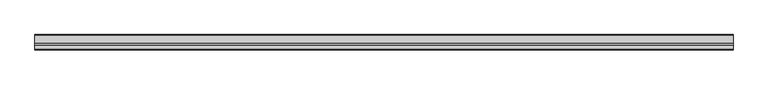
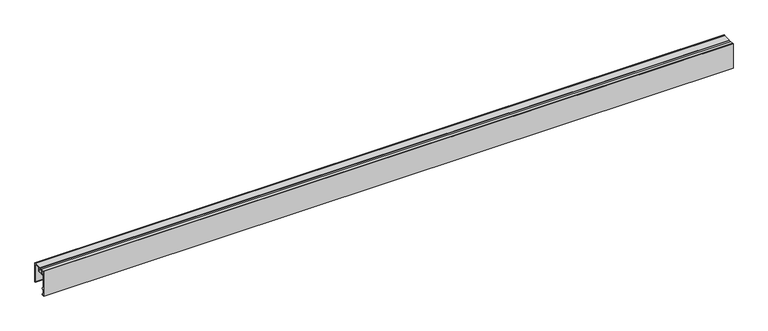
"""IFC4 building model written with IfcOpenShell, lengths in millimetres: proxy geometry, Generic Models 6:Generic Models 2:318829:Generic Models 2:318829 : Generic Models 6:Generic Models 2:318829:2 : Generic Models 6:Generic Models 2:318829:Generic Models 2:318829 : Generic Models 6:Generic Models 2:318829:300683."""

from ifc_helpers import new_model, si_unit, frame, origin, place, context, project, spatial, polyline, outline, extrude, source, transform, mapped, element, save


def generic_models_cac01c20(model_context):
    return source(origin(), model_context, "Body", "SweptSolid", [
        extrude(outline(polyline([(-536491.165958, 10109.8070812), (-536491.165958, 10105.1095826), (-536493.0913734, 10105.1095826), (-536493.0913734, 10102.7283326), (-536491.165958, 10102.7283326), (-536491.165958, 10098.030834), (-536507.7182141, 10098.030834), (-536507.7182141, 10102.7283326), (-536505.7927987, 10102.7283326), (-536505.7927987, 10105.1095826), (-536507.7182141, 10105.1095826), (-536507.7182141, 10109.8070812), (-536491.165958, 10109.8070812)])), frame((591391.6367242, 0.0, 0.0), z_axis=(1.0, 0.0, 0.0), x_axis=(0.0, 1.0, 0.0)), (0.0, 0.0, 1.0), 2438.4),
        extrude(outline(polyline([(-536517.6457241, 10111.7914562), (-536503.9479016, 10111.7914562), (-536503.9479016, 10110.2039562), (-536508.1150891, 10110.2039562), (-536508.1150891, 10104.7127076), (-536506.1896737, 10104.7127076), (-536506.1896737, 10103.1252076), (-536508.1150891, 10103.1252076), (-536508.1150891, 10097.633959), (-536503.9479016, 10097.633959), (-536503.9479016, 10096.046459), (-536517.6457241, 10096.046459), (-536517.6457241, 10044.5539562), (-536512.3743526, 10044.5539562), (-536512.3743526, 10047.3537828), (-536510.7868526, 10047.3537828), (-536510.7868526, 10042.9664562), (-536517.6457241, 10042.9664562), (-536517.6457241, 10022.9664562), (-536512.3743526, 10022.9664562), (-536512.3743526, 10025.7662828), (-536510.7868526, 10025.7662828), (-536510.7868526, 10021.3789562), (-536519.2332241, 10021.3789562), (-536519.2332241, 10113.3789562), (-536517.6457241, 10113.3789562), (-536517.6457241, 10111.7914562)]), holes=[polyline([(-536517.6457241, 10097.633959), (-536509.7025891, 10097.633959), (-536509.7025891, 10110.2039562), (-536517.6457241, 10110.2039562), (-536517.6457241, 10097.633959)])]), frame((591391.6367242, 0.0, 0.0), z_axis=(1.0, 0.0, 0.0), x_axis=(0.0, 1.0, 0.0)), (0.0, 0.0, 1.0), 2438.4),
        extrude(outline(polyline([(-536467.9483141, 10042.9664562), (-536466.8207241, 10042.9664562), (-536466.8207241, 10110.2039562), (-536489.181583, 10110.2039562), (-536489.181583, 10096.046459), (-536494.9362705, 10096.046459), (-536494.9362705, 10097.633959), (-536490.769083, 10097.633959), (-536490.769083, 10103.1252076), (-536492.6944984, 10103.1252076), (-536492.6944984, 10104.7127076), (-536490.769083, 10104.7127076), (-536490.769083, 10110.2039562), (-536494.9362705, 10110.2039562), (-536494.9362705, 10111.7914562), (-536466.8207241, 10111.7914562), (-536466.8207241, 10113.3789562), (-536465.2332241, 10113.3789562), (-536465.2332241, 10041.3789562), (-536467.9483141, 10041.3789562), (-536467.9483141, 10042.9664562)])), frame((591391.6367242, 0.0, 0.0), z_axis=(1.0, 0.0, 0.0), x_axis=(0.0, 1.0, 0.0)), (0.0, 0.0, 1.0), 2438.4),
    ])


if __name__ == "__main__":
    model = new_model("IFC4")
    model_context = context("Model", 3, world=origin())
    ifc_project = project(units=[si_unit("LENGTHUNIT", "METRE", prefix="MILLI")], contexts=[model_context])
    site = spatial("IfcSite", under=ifc_project)
    building = spatial("IfcBuilding", under=site)
    placement = place(None, origin())
    generic_models_shape = generic_models_cac01c20(model_context)
    element("IfcBuildingElementProxy", 1, Name="Generic Models 6:Generic Models 2:318829:Generic Models 2:318829 : Generic Models 6:Generic Models 2:318829:2 : Generic Models 6:Generic Models 2:318829:Generic Models 2:318829 : Generic Models 6:Generic Models 2:318829:300683", ObjectType="Generic Models 6:Generic Models 2:318829:Generic Models 2:318829 : Generic Models 6:Generic Models 2:318829:2 : Generic Models 6:Generic Models 2:318829:Generic Models 2:318829 : Generic Models 6:Generic Models 2:318829:300683", at=placement, inside=building, context=model_context, shape_type="MappedRepresentation", body=[
        mapped(generic_models_shape, transform((0.0, 0.0, 0.0), x_axis=(1.0, 0.0, 0.0), y_axis=(0.0, 1.0, 0.0), z_axis=(0.0, 0.0, 1.0))),
    ])
    save(model, "model.ifc")

# Revit data of these elements
# Type "Generic Models 6:Generic Models 2:318829:Generic Models 2:318829 : Generic Models 6:Generic Models 2:318829:2 : Generic Models 6:Generic Models 2:318829:Generic Models 2:318829 : Generic Models 6:Generic Models 2:318829:300683"
#   NameOverride = "Generic Models 6:Generic Models 2:318829:Generic Models 2:318829 : Generic Models 6:Generic Models 2:318829:300683"
#   ObjectTypeOverride = "Generic Models 2:318829 : Generic Models 6:Generic Models 2:318829"
#   Reference = "Generic Models 2"
#   Tag = "300683"
# Element 1 (IfcBuildingElementProxy, "Generic Models 6:Generic Models 2:318829:Generic Models 2:318829 : Generic Models 6:Generic Models 2:318829:2 : Generic Models 6:Generic Models 2:318829:Generic Models 2:318829 : Generic Models 6:Generic Models 2:318829:300683")
#   Materials on its faces: "THERMAL BROKEN ALUMINUM STOREFRONT FOR POLYCARBONATE"
# Materials
#   "THERMAL BROKEN ALUMINUM STOREFRONT FOR POLYCARBONATE": class "Unassigned", colour RGB 244 244 244, transparency 0, Keynote = "M07611300.01", Cost = 0
